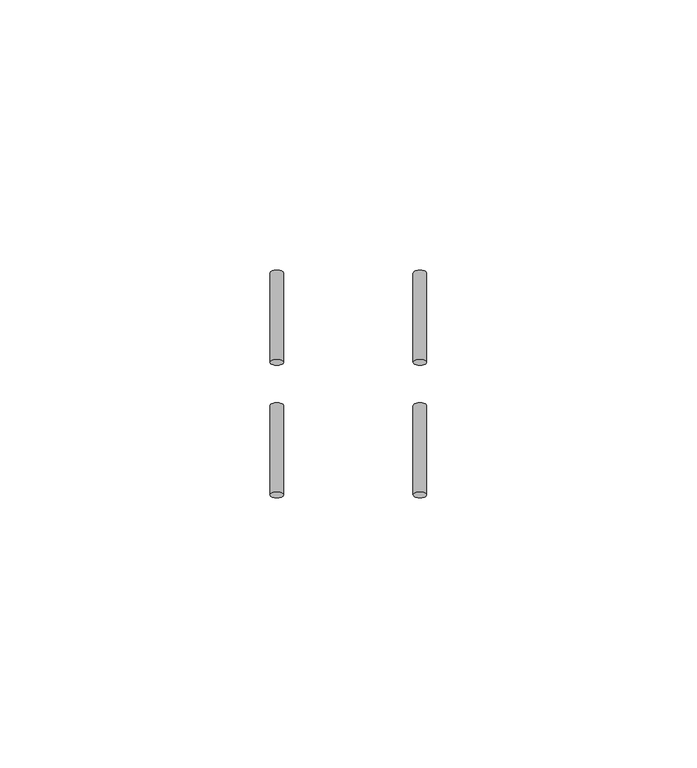
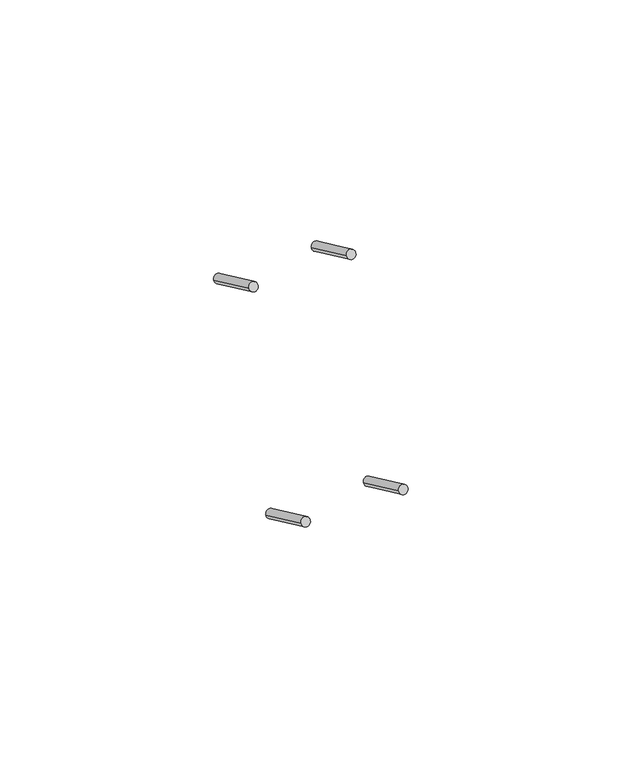
"""IFC4 building model written with IfcOpenShell, lengths in millimetres: furniture geometry, MOLDURA TELA2 : MOLDURA TELA."""

import ifcopenshell
import ifcopenshell.guid

model = None  # the IFC model being written
_history = None  # IfcOwnerHistory: only IFC2X3 demands one
_inside = {}  # id of a spatial element -> (the spatial element, [elements in it])
_under = {}  # id of a project, library or spatial element -> (it, [spatial elements below it])
_declared = {}  # id of a project -> (the project, [libraries it declares])
_typed = {}  # id of a type object -> (the type object, [elements of that type])
_made_of = {}  # id of a material, layer set ... -> (it, [elements and type objects made of it])


def new_model(schema):
    """Start an empty IFC model of exactly this schema.

    Asked for "IFC4X3", IfcOpenShell would pick the latest addendum, in which some entities
    have other attributes; the version numbers below select the first issue.
    IFC2X3 requires an IfcOwnerHistory on every rooted entity: one is made here for all.
    """
    global model, _history
    if schema == "IFC4X3":
        model = ifcopenshell.file(schema_version=(4, 3, 0, 0))
    else:
        model = ifcopenshell.file(schema=schema)
    _inside.clear()
    _under.clear()
    _declared.clear()
    _typed.clear()
    _made_of.clear()
    _history = None
    if model.schema == "IFC2X3":
        org = make("IfcOrganization", Name="unknown")
        user = make(
            "IfcPersonAndOrganization",
            ThePerson=make("IfcPerson", FamilyName="unknown"),
            TheOrganization=org,
        )
        app = make(
            "IfcApplication",
            ApplicationDeveloper=org,
            Version="unknown",
            ApplicationFullName="unknown",
            ApplicationIdentifier="unknown",
        )
        _history = make(
            "IfcOwnerHistory",
            OwningUser=user,
            OwningApplication=app,
            ChangeAction="ADDED",
            CreationDate=0,
        )
    return model


def make(cls, **values):
    """One entity of the class cls with the attributes given. An attribute that is None is left unset."""
    return model.create_entity(
        cls, **{name: value for name, value in values.items() if value is not None}
    )


def rooted(cls, **values):
    """An entity with a GlobalId (a new one), such as an element, a storey or a relation."""
    return make(cls, GlobalId=ifcopenshell.guid.new(), OwnerHistory=_history, **values)


def si_unit(unit_type, name, prefix=None):
    """IfcSIUnit, for example si_unit("LENGTHUNIT", "METRE", prefix="MILLI")."""
    return make("IfcSIUnit", UnitType=unit_type, Prefix=prefix, Name=name)


def assignment(units):
    """IfcUnitAssignment: the units of a project."""
    return None if units is None else make("IfcUnitAssignment", Units=units)


def point(xyz):
    """IfcCartesianPoint."""
    return None if xyz is None else make("IfcCartesianPoint", Coordinates=xyz)


def direction(xyz):
    """IfcDirection."""
    return None if xyz is None else make("IfcDirection", DirectionRatios=xyz)


def frame(location, z_axis=None, x_axis=None):
    """IfcAxis2Placement3D, a coordinate frame: its origin and axes. An axis left out is left unset."""
    return make(
        "IfcAxis2Placement3D",
        Location=point(location),
        Axis=direction(z_axis),
        RefDirection=direction(x_axis),
    )


def frame_2d(location, x_axis=None):
    """IfcAxis2Placement2D, a coordinate frame in the plane: its origin and x axis."""
    return make(
        "IfcAxis2Placement2D", Location=point(location), RefDirection=direction(x_axis)
    )


def origin():
    """The frame at (0, 0, 0) with its axes left unset."""
    return frame((0.0, 0.0, 0.0))


def place(relative_to, where):
    """IfcLocalPlacement: puts the frame where relative to a parent placement (None: the world)."""
    return make(
        "IfcLocalPlacement", PlacementRelTo=relative_to, RelativePlacement=where
    )


def context(
    kind, dimensions, precision=None, world=None, true_north=None, identifier=None
):
    """IfcGeometricRepresentationContext, for example the 3D "Model" context."""
    return make(
        "IfcGeometricRepresentationContext",
        ContextIdentifier=identifier,
        ContextType=kind,
        CoordinateSpaceDimension=dimensions,
        Precision=precision,
        WorldCoordinateSystem=world,
        TrueNorth=true_north,
    )


def project(units=None, contexts=None):
    """IfcProject with its units and contexts."""
    return rooted(
        "IfcProject",
        Name="project",
        RepresentationContexts=contexts,
        UnitsInContext=assignment(units),
    )


def spatial(cls, under=None, at=None, **own):
    """A site, building, storey or space (cls), placed at a placement, below another one or the project."""
    s = rooted(cls, ObjectPlacement=at, **own)
    if under is not None:
        _under.setdefault(under.id(), (under, []))[1].append(s)
    return s


def circle_curve(where, radius):
    """IfcCircle in the frame where."""
    return make("IfcCircle", Position=where, Radius=radius)


def trimmed(basis, trim1, trim2, sense, master):
    """IfcTrimmedCurve: the piece of a basis curve between two trims."""
    return make(
        "IfcTrimmedCurve",
        BasisCurve=basis,
        Trim1=trim1,
        Trim2=trim2,
        SenseAgreement=sense,
        MasterRepresentation=master,
    )


def segment(curve, same_sense, transition):
    """IfcCompositeCurveSegment."""
    return make(
        "IfcCompositeCurveSegment",
        Transition=transition,
        SameSense=same_sense,
        ParentCurve=curve,
    )


def composite_curve(segments, self_intersect=None):
    """IfcCompositeCurve: segments joined end to end."""
    return make("IfcCompositeCurve", Segments=segments, SelfIntersect=self_intersect)


def outline(outer, holes=None, kind="AREA"):
    """IfcArbitraryClosedProfileDef: a profile drawn as a closed curve; with holes, ...WithVoids."""
    if holes is None:
        return make("IfcArbitraryClosedProfileDef", ProfileType=kind, OuterCurve=outer)
    return make(
        "IfcArbitraryProfileDefWithVoids",
        ProfileType=kind,
        OuterCurve=outer,
        InnerCurves=holes,
    )


def extrude(swept, where, along, depth):
    """IfcExtrudedAreaSolid: the profile swept, set in the frame where, extruded along a direction by depth."""
    return make(
        "IfcExtrudedAreaSolid",
        SweptArea=swept,
        Position=where,
        ExtrudedDirection=direction(along),
        Depth=depth,
    )


def shape(context_of_items, identifier, shape_type, items):
    """IfcShapeRepresentation: the items that make up one representation, for example the "Body"."""
    return make(
        "IfcShapeRepresentation",
        ContextOfItems=context_of_items,
        RepresentationIdentifier=identifier,
        RepresentationType=shape_type,
        Items=items,
    )


def source(mapping_origin, context_of_items, identifier, shape_type, items):
    """IfcRepresentationMap: a shape defined once, which mapped items show again and again."""
    return make(
        "IfcRepresentationMap",
        MappingOrigin=mapping_origin,
        MappedRepresentation=shape(context_of_items, identifier, shape_type, items),
    )


def transform(
    local_origin,
    x_axis=None,
    y_axis=None,
    z_axis=None,
    scale=None,
    scale2=None,
    scale3=None,
    uniform=True,
):
    """IfcCartesianTransformationOperator3D, or its non-uniform kind. x_axis, y_axis, z_axis: its Axis1, 2, 3."""
    if uniform:
        return make(
            "IfcCartesianTransformationOperator3D",
            Axis1=direction(x_axis),
            Axis2=direction(y_axis),
            LocalOrigin=point(local_origin),
            Scale=scale,
            Axis3=direction(z_axis),
        )
    return make(
        "IfcCartesianTransformationOperator3DnonUniform",
        Axis1=direction(x_axis),
        Axis2=direction(y_axis),
        LocalOrigin=point(local_origin),
        Scale=scale,
        Axis3=direction(z_axis),
        Scale2=scale2,
        Scale3=scale3,
    )


def mapped(mapping_source, mapping_target):
    """IfcMappedItem: shows the shape of a source again, moved by a transform."""
    return make(
        "IfcMappedItem", MappingSource=mapping_source, MappingTarget=mapping_target
    )


def made_of(thing, what):
    """Note that an element or type object is made of a material, layer set ...; save() writes the relation."""
    if what is not None:
        _made_of.setdefault(what.id(), (what, []))[1].append(thing)
    return thing


def element(
    cls,
    number,
    at=None,
    inside=None,
    cuts=None,
    type_object=None,
    material=None,
    context=None,
    identifier="Body",
    shape_type=None,
    held_by="IfcProductDefinitionShape",
    body=None,
    shapes=None,
    **own,
):
    """One element of the class cls, such as IfcWall. Its Tag is "e" and its number.

    at: its placement. inside: the storey or other place that contains it. cuts: it is an
    opening in that element (IfcRelVoidsElement). A single representation is given by context,
    identifier, shape_type and body (its items); several are given by shapes. held_by: the class
    of the entity that holds the representations. save() writes the other relations.
    """
    e = rooted(cls, Tag="e%d" % number, ObjectPlacement=at, **own)
    if body is not None:
        shapes = [shape(context, identifier, shape_type, body)]
    if shapes is not None:
        e.Representation = make(held_by, Representations=shapes)
    if inside is not None:
        _inside.setdefault(inside.id(), (inside, []))[1].append(e)
    if cuts is not None:
        rooted(
            "IfcRelVoidsElement", RelatingBuildingElement=cuts, RelatedOpeningElement=e
        )
    if type_object is not None:
        _typed.setdefault(type_object.id(), (type_object, []))[1].append(e)
    return made_of(e, material)


def aggregate(whole, parts):
    """IfcRelAggregates: a whole, such as a stair, and the parts it consists of."""
    return rooted("IfcRelAggregates", RelatingObject=whole, RelatedObjects=parts)


def save(model, path):
    """Write the relations noted so far, then the file.

    IfcRelAggregates (storeys below a building ...), IfcRelContainedInSpatialStructure (elements
    in a storey), IfcRelDefinesByType, IfcRelAssociatesMaterial and IfcRelDeclares: one each for
    every whole, place, type object, material and project.
    """
    for whole, parts in _under.values():
        aggregate(whole, parts)
    for where, things in _inside.values():
        rooted(
            "IfcRelContainedInSpatialStructure",
            RelatedElements=things,
            RelatingStructure=where,
        )
    for kind, things in _typed.values():
        rooted("IfcRelDefinesByType", RelatedObjects=things, RelatingType=kind)
    for what, things in _made_of.values():
        rooted("IfcRelAssociatesMaterial", RelatedObjects=things, RelatingMaterial=what)
    for by, libraries in _declared.values():
        rooted("IfcRelDeclares", RelatingContext=by, RelatedDefinitions=libraries)
    model.write(path)


def furniture_6f4f2263(model_context):
    return source(origin(), model_context, "Body", "SweptSolid", [
        extrude(outline(composite_curve([segment(trimmed(circle_curve(frame_2d((0.0, -1.25)), 1.25), [point((0.0, 0.0))], [point((0.0, -2.5))], False, "CARTESIAN"), True, "CONTINUOUS"), segment(trimmed(circle_curve(frame_2d((0.0, -1.25)), 1.25), [point((0.0, -2.5))], [point((0.0, 0.0))], False, "CARTESIAN"), True, "CONTINUOUS")], self_intersect=False)), frame((2402.7219295, 1333.1379685, 54.4576905), z_axis=(0.0, -0.9063077870366535, 0.4226182617406919), x_axis=(0.0, 0.4226182617406919, 0.9063077870366535)), (0.0, 0.0, 1.0), 18.2226949),
        extrude(outline(composite_curve([segment(trimmed(circle_curve(frame_2d((-58.0000001, -1.25)), 1.25), [point((-58.0000001, -2.5))], [point((-58.0000001, 0.0))], False, "CARTESIAN"), True, "CONTINUOUS"), segment(trimmed(circle_curve(frame_2d((-58.0000001, -1.25)), 1.25), [point((-58.0000001, 0.0))], [point((-58.0000001, -2.5))], False, "CARTESIAN"), True, "CONTINUOUS")], self_intersect=False)), frame((2402.7219295, 1333.1379685, 54.4576905), z_axis=(0.0, -0.9063077870366535, 0.4226182617406919), x_axis=(0.0, 0.4226182617406919, 0.9063077870366535)), (0.0, 0.0, 1.0), 18.2226949),
        extrude(outline(composite_curve([segment(trimmed(circle_curve(frame_2d((-58.0000001, 25.25)), 1.25), [point((-58.0000001, 24.0))], [point((-58.0000001, 26.5))], False, "CARTESIAN"), True, "CONTINUOUS"), segment(trimmed(circle_curve(frame_2d((-58.0000001, 25.25)), 1.25), [point((-58.0000001, 26.5))], [point((-58.0000001, 24.0))], False, "CARTESIAN"), True, "CONTINUOUS")], self_intersect=False)), frame((2402.7219295, 1333.1379685, 54.4576905), z_axis=(0.0, -0.9063077870366535, 0.4226182617406919), x_axis=(0.0, 0.4226182617406919, 0.9063077870366535)), (0.0, 0.0, 1.0), 18.2226949),
        extrude(outline(composite_curve([segment(trimmed(circle_curve(frame_2d((0.0, 25.25)), 1.25), [point((0.0, 24.0))], [point((0.0, 26.5))], False, "CARTESIAN"), True, "CONTINUOUS"), segment(trimmed(circle_curve(frame_2d((0.0, 25.25)), 1.25), [point((0.0, 26.5))], [point((0.0, 24.0))], False, "CARTESIAN"), True, "CONTINUOUS")], self_intersect=False)), frame((2402.7219295, 1333.1379685, 54.4576905), z_axis=(0.0, -0.9063077870366535, 0.4226182617406919), x_axis=(0.0, 0.4226182617406919, 0.9063077870366535)), (0.0, 0.0, 1.0), 18.2226949),
    ])


if __name__ == "__main__":
    model = new_model("IFC4")
    model_context = context("Model", 3, world=origin())
    ifc_project = project(units=[si_unit("LENGTHUNIT", "METRE", prefix="MILLI")], contexts=[model_context])
    site = spatial("IfcSite", under=ifc_project)
    building = spatial("IfcBuilding", under=site)
    placement = place(None, origin())
    furniture_shape = furniture_6f4f2263(model_context)
    element("IfcFurniture", 1, ObjectType="MOLDURA TELA2 : MOLDURA TELA", at=placement, inside=building, context=model_context, shape_type="MappedRepresentation", body=[
        mapped(furniture_shape, transform((0.0, 0.0, 0.0), x_axis=(1.0, 0.0, 0.0), y_axis=(0.0, 1.0, 0.0), z_axis=(0.0, 0.0, 1.0))),
    ])
    save(model, "model.ifc")

# Revit data of these elements
# Type "MOLDURA TELA2 : MOLDURA TELA"
#   Height = 0
# Element 1 (IfcFurniture, "MOLDURA TELA2 : MOLDURA TELA")
#   Materials on its faces: "Aço, Carbono"
# Materials
#   "Aço, Carbono": class "Metal", colour RGB 0 0 0, transparency 0, Description = "Aço Carbono", Cost = 0
